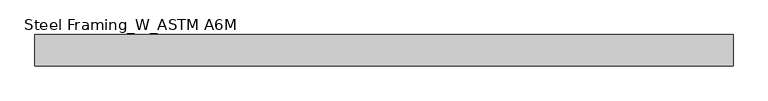
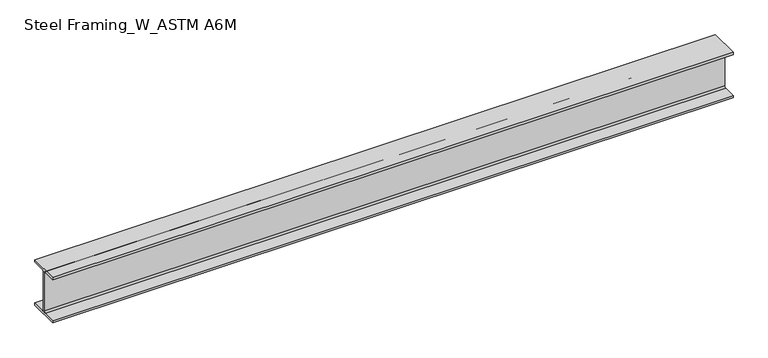
"""IFC4 building model written with IfcOpenShell, lengths in millimetres: beam geometry, Steel Framing_W_ASTM A6M : H_SB_AR_S02_W200x31.3_B6."""

from ifc_helpers import new_model, si_unit, point, frame, frame_2d, origin, place, context, project, spatial, polyline, circle_curve, trimmed, segment, composite_curve, outline, extrude, source, transform, mapped, element, save


def steel_framing_w_astm_a6m_95b0337f(model_context):
    return source(origin(), model_context, "Body", "SweptSolid", [
        extrude(outline(composite_curve([segment(polyline([(67.0, -94.8), (67.0, -105.0), (-67.0, -105.0), (-67.0, -94.8), (-10.775, -94.8)]), True, "CONTINUOUS"), segment(trimmed(circle_curve(frame_2d((-10.775, -87.2)), 7.6), [point((-10.775, -94.8))], [point((-3.175, -87.2))], True, "CARTESIAN"), True, "CONTINUOUS"), segment(polyline([(-3.175, -87.2), (-3.175, 87.2)]), True, "CONTINUOUS"), segment(trimmed(circle_curve(frame_2d((-10.775, 87.2)), 7.6), [point((-3.175, 87.2))], [point((-10.775, 94.8))], True, "CARTESIAN"), True, "CONTINUOUS"), segment(polyline([(-10.775, 94.8), (-67.0, 94.8), (-67.0, 105.0), (67.0, 105.0), (67.0, 94.8), (10.775, 94.8)]), True, "CONTINUOUS"), segment(trimmed(circle_curve(frame_2d((10.775, 87.2)), 7.6), [point((10.775, 94.8))], [point((3.175, 87.2))], True, "CARTESIAN"), True, "CONTINUOUS"), segment(polyline([(3.175, 87.2), (3.175, -87.2)]), True, "CONTINUOUS"), segment(trimmed(circle_curve(frame_2d((10.775, -87.2)), 7.6), [point((3.175, -87.2))], [point((10.775, -94.8))], True, "CARTESIAN"), True, "CONTINUOUS"), segment(polyline([(10.775, -94.8), (67.0, -94.8)]), True, "CONTINUOUS")], self_intersect=False)), frame((-1487.2, 0.0, 0.0), z_axis=(1.0, 0.0, 0.0), x_axis=(0.0, 1.0, 0.0)), (0.0, 0.0, 1.0), 2974.4),
    ])


if __name__ == "__main__":
    model = new_model("IFC4")
    model_context = context("Model", 3, world=origin())
    ifc_project = project(units=[si_unit("LENGTHUNIT", "METRE", prefix="MILLI")], contexts=[model_context])
    site = spatial("IfcSite", under=ifc_project)
    building = spatial("IfcBuilding", under=site)
    placement = place(None, origin())
    steel_framing_w_astm_a6m_shape = steel_framing_w_astm_a6m_95b0337f(model_context)
    element("IfcBeam", 1, ObjectType="Steel Framing_W_ASTM A6M : H_SB_AR_S02_W200x31.3_B6", at=placement, inside=building, context=model_context, shape_type="MappedRepresentation", body=[
        mapped(steel_framing_w_astm_a6m_shape, transform((0.0, 0.0, 0.0), x_axis=(1.0, 0.0, 0.0), y_axis=(0.0, 1.0, 0.0), z_axis=(0.0, 0.0, 1.0))),
    ])
    save(model, "model.ifc")

# Revit data of these elements
# Type "Steel Framing_W_ASTM A6M : H_SB_AR_S02_W200x31.3_B6"
#   Type Mark = "B6"
#   Section Name Key = "W8x21"
#   Width = 13.4 cm
#   Web Thickness = 0.635 cm
#   Web Fillet = 0.76 cm
#   Warping Constant = 40800.0 cm⁶
#   Torsional Moment of Inertia = 11.70 cm⁴
#   Section Area = 39.7 cm²
#   Plastic Modulus weak axis = 93.2 cm³
#   Plastic Modulus strong axis = 334.0 cm³
#   Perimeter = 0.93 m²/m
#   Nominal Weight = 31.30 kgf/m
#   Moment of Inertia weak axis = 407.00 cm⁴
#   Moment of Inertia strong axis = 3130.00 cm⁴
#   Height = 21.0 cm
#   Flange Thickness = 1.02 cm
#   Elastic Modulus weak axis = 60.8 cm³
#   Elastic Modulus strong axis = 298.0 cm³
#   Centroid Vertical = 10.5 cm
#   Centroid Horizontal = 6.7 cm
#   Length [instance default] = 1500 mm
#   Structural Material [instance default] = Steel, 45-345
#   Bolt Spacing = 0
#   Assembly Code = ""
# Element 1 (IfcBeam, "Steel Framing_W_ASTM A6M : H_SB_AR_S02_W200x31.3_B6")
#   Materials on its faces: "Steel, 45-345"
# Materials
#   "Steel, 45-345": class "Metal", colour RGB 189 187 185, transparency 0, Description = "Steel 345 MPa", Cost = 0
